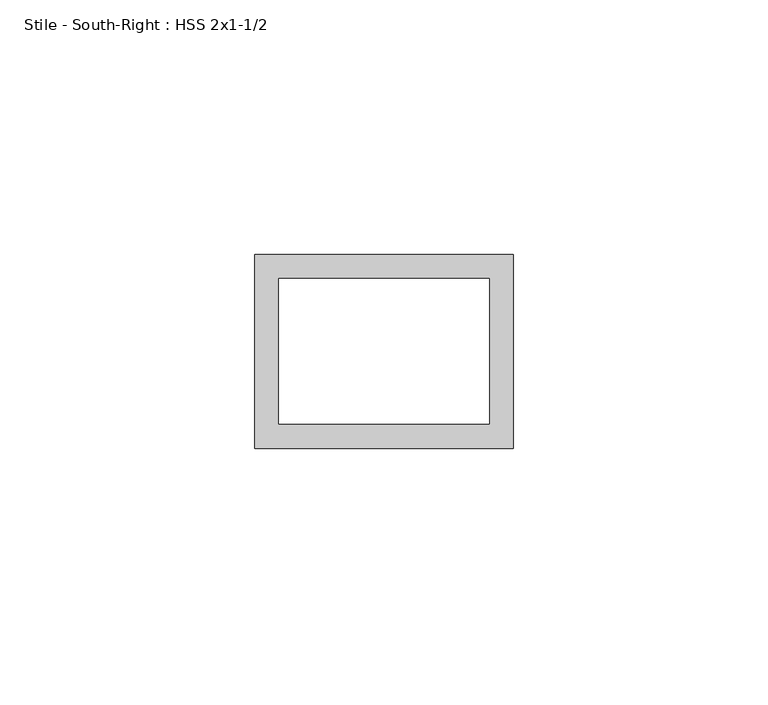
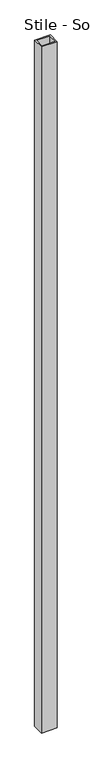
"""IFC4 building model written with IfcOpenShell, lengths in millimetres: proxy geometry, Stile - South-Right : HSS 2x1-1/2."""

from ifc_helpers import new_model, si_unit, frame, origin, place, context, project, spatial, polyline, outline, extrude, source, transform, mapped, element, save


def stile_south_right_hss_2x1_1_2_5f68abb1(model_context):
    return source(origin(), model_context, "Body", "SweptSolid", [
        extrude(outline(polyline([(587365.8934739, -533937.9163841), (587416.6934739, -533937.9163841), (587416.6934739, -533976.0163841), (587365.8934739, -533976.0163841), (587365.8934739, -533937.9163841)]), holes=[polyline([(587370.6559739, -533942.6788841), (587370.6559739, -533971.2538841), (587411.9309739, -533971.2538841), (587411.9309739, -533942.6788841), (587370.6559739, -533942.6788841)])]), frame((0.0, 0.0, 50.8), z_axis=(0.0, 0.0, 1.0), x_axis=(1.0, 0.0, 0.0)), (0.0, 0.0, 1.0), 2349.5),
    ])


if __name__ == "__main__":
    model = new_model("IFC4")
    model_context = context("Model", 3, world=origin())
    ifc_project = project(units=[si_unit("LENGTHUNIT", "METRE", prefix="MILLI")], contexts=[model_context])
    site = spatial("IfcSite", under=ifc_project)
    building = spatial("IfcBuilding", under=site)
    placement = place(None, origin())
    stile_south_right_hss_2x1_1_2_shape = stile_south_right_hss_2x1_1_2_5f68abb1(model_context)
    element("IfcBuildingElementProxy", 1, Name="Stile - South-Right : HSS 2x1-1/2", ObjectType="Stile - South-Right : HSS 2x1-1/2", at=placement, inside=building, context=model_context, shape_type="MappedRepresentation", body=[
        mapped(stile_south_right_hss_2x1_1_2_shape, transform((0.0, 0.0, 0.0), x_axis=(1.0, 0.0, 0.0), y_axis=(0.0, 1.0, 0.0), z_axis=(0.0, 0.0, 1.0))),
    ])
    save(model, "model.ifc")

# Revit data of these elements
# Element 1 (IfcBuildingElementProxy, "Stile - South-Right : HSS 2x1-1/2")
#   Materials on its faces: "1-1/2\"X2\" GALV. STL HSS TUBING"
# Materials
#   "1-1/2\"X2\" GALV. STL HSS TUBING": class "Generic", colour RGB 211 211 207, transparency 0, Cost = 0
